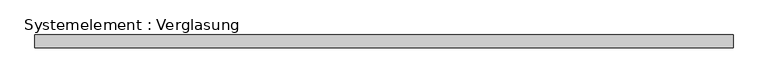
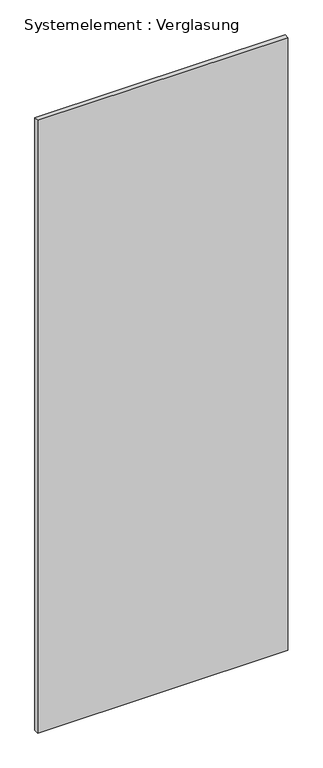
"""IFC4 building model written with IfcOpenShell, lengths in millimetres: plate geometry, Systemelement : Verglasung."""

from ifc_helpers import new_model, si_unit, origin, origin_with_axes, place, context, project, spatial, polyline, outline, extrude, source, transform, mapped, element, save


def systemelement_verglasung_0d66f548(model_context):
    return source(origin(), model_context, "Body", "SweptSolid", [
        extrude(outline(polyline([(818.3124796, -15.0), (-818.3124796, -15.0), (-818.3124796, 15.0), (818.3124796, 15.0), (818.3124796, -15.0)])), origin_with_axes(), (0.0, 0.0, 1.0), 4236.6788019),
    ])


if __name__ == "__main__":
    model = new_model("IFC4")
    model_context = context("Model", 3, world=origin())
    ifc_project = project(units=[si_unit("LENGTHUNIT", "METRE", prefix="MILLI")], contexts=[model_context])
    site = spatial("IfcSite", under=ifc_project)
    building = spatial("IfcBuilding", under=site)
    placement = place(None, origin())
    systemelement_verglasung_shape = systemelement_verglasung_0d66f548(model_context)
    element("IfcPlate", 1, ObjectType="Systemelement : Verglasung", at=placement, inside=building, context=model_context, shape_type="MappedRepresentation", body=[
        mapped(systemelement_verglasung_shape, transform((0.0, 0.0, 0.0), x_axis=(1.0, 0.0, 0.0), y_axis=(0.0, 1.0, 0.0), z_axis=(0.0, 0.0, 1.0))),
    ])
    save(model, "model.ifc")

# Revit data of these elements
# Type "Systemelement : Verglasung"
#   Construction Type Id = "GSP4R"
#   Analytic Construction = "1/8 Zoll Pilkington-Verglasung einfach"
#   Visual Light Transmittance = 0.9
#   Solar Heat Gain Coefficient = 0.86
#   Heat Transfer Coefficient (U) = 6.7069 W/(m²·K)
# Element 1 (IfcPlate, "Systemelement : Verglasung")
#   Materials on its faces: "Glas"
# Materials
#   "Glas": class "Glas", colour RGB 0 0 255, transparency 0.75, Comments = "Render-Darstellung nicht aktualisiert ", Cost = 0
